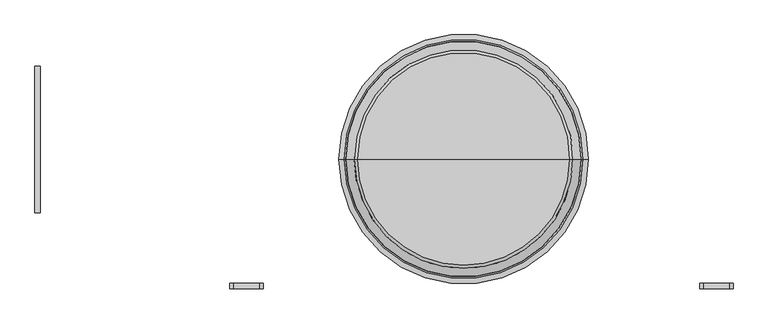
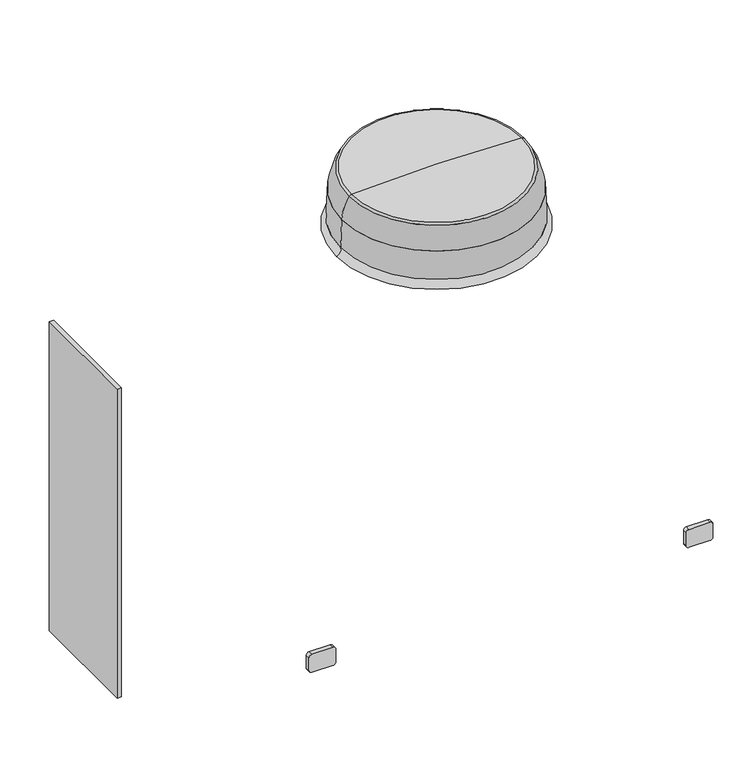
"""IFC4 building model written with IfcOpenShell, lengths in millimetres: proxy geometry, PURY-P168-288_YSJMU_Heat_Recovery_460V : PURY-P192YSJMU-A(-BS)_460V."""

import ifcopenshell
import ifcopenshell.guid

model = None  # the IFC model being written
_history = None  # IfcOwnerHistory: only IFC2X3 demands one
_inside = {}  # id of a spatial element -> (the spatial element, [elements in it])
_under = {}  # id of a project, library or spatial element -> (it, [spatial elements below it])
_declared = {}  # id of a project -> (the project, [libraries it declares])
_typed = {}  # id of a type object -> (the type object, [elements of that type])
_made_of = {}  # id of a material, layer set ... -> (it, [elements and type objects made of it])


def new_model(schema):
    """Start an empty IFC model of exactly this schema.

    Asked for "IFC4X3", IfcOpenShell would pick the latest addendum, in which some entities
    have other attributes; the version numbers below select the first issue.
    IFC2X3 requires an IfcOwnerHistory on every rooted entity: one is made here for all.
    """
    global model, _history
    if schema == "IFC4X3":
        model = ifcopenshell.file(schema_version=(4, 3, 0, 0))
    else:
        model = ifcopenshell.file(schema=schema)
    _inside.clear()
    _under.clear()
    _declared.clear()
    _typed.clear()
    _made_of.clear()
    _history = None
    if model.schema == "IFC2X3":
        org = make("IfcOrganization", Name="unknown")
        user = make(
            "IfcPersonAndOrganization",
            ThePerson=make("IfcPerson", FamilyName="unknown"),
            TheOrganization=org,
        )
        app = make(
            "IfcApplication",
            ApplicationDeveloper=org,
            Version="unknown",
            ApplicationFullName="unknown",
            ApplicationIdentifier="unknown",
        )
        _history = make(
            "IfcOwnerHistory",
            OwningUser=user,
            OwningApplication=app,
            ChangeAction="ADDED",
            CreationDate=0,
        )
    return model


def make(cls, **values):
    """One entity of the class cls with the attributes given. An attribute that is None is left unset."""
    return model.create_entity(
        cls, **{name: value for name, value in values.items() if value is not None}
    )


def rooted(cls, **values):
    """An entity with a GlobalId (a new one), such as an element, a storey or a relation."""
    return make(cls, GlobalId=ifcopenshell.guid.new(), OwnerHistory=_history, **values)


def si_unit(unit_type, name, prefix=None):
    """IfcSIUnit, for example si_unit("LENGTHUNIT", "METRE", prefix="MILLI")."""
    return make("IfcSIUnit", UnitType=unit_type, Prefix=prefix, Name=name)


def assignment(units):
    """IfcUnitAssignment: the units of a project."""
    return None if units is None else make("IfcUnitAssignment", Units=units)


def point(xyz):
    """IfcCartesianPoint."""
    return None if xyz is None else make("IfcCartesianPoint", Coordinates=xyz)


def direction(xyz):
    """IfcDirection."""
    return None if xyz is None else make("IfcDirection", DirectionRatios=xyz)


def frame(location, z_axis=None, x_axis=None):
    """IfcAxis2Placement3D, a coordinate frame: its origin and axes. An axis left out is left unset."""
    return make(
        "IfcAxis2Placement3D",
        Location=point(location),
        Axis=direction(z_axis),
        RefDirection=direction(x_axis),
    )


def frame_2d(location, x_axis=None):
    """IfcAxis2Placement2D, a coordinate frame in the plane: its origin and x axis."""
    return make(
        "IfcAxis2Placement2D", Location=point(location), RefDirection=direction(x_axis)
    )


def origin():
    """The frame at (0, 0, 0) with its axes left unset."""
    return frame((0.0, 0.0, 0.0))


def place(relative_to, where):
    """IfcLocalPlacement: puts the frame where relative to a parent placement (None: the world)."""
    return make(
        "IfcLocalPlacement", PlacementRelTo=relative_to, RelativePlacement=where
    )


def context(
    kind, dimensions, precision=None, world=None, true_north=None, identifier=None
):
    """IfcGeometricRepresentationContext, for example the 3D "Model" context."""
    return make(
        "IfcGeometricRepresentationContext",
        ContextIdentifier=identifier,
        ContextType=kind,
        CoordinateSpaceDimension=dimensions,
        Precision=precision,
        WorldCoordinateSystem=world,
        TrueNorth=true_north,
    )


def project(units=None, contexts=None):
    """IfcProject with its units and contexts."""
    return rooted(
        "IfcProject",
        Name="project",
        RepresentationContexts=contexts,
        UnitsInContext=assignment(units),
    )


def spatial(cls, under=None, at=None, **own):
    """A site, building, storey or space (cls), placed at a placement, below another one or the project."""
    s = rooted(cls, ObjectPlacement=at, **own)
    if under is not None:
        _under.setdefault(under.id(), (under, []))[1].append(s)
    return s


def polyline(points):
    """IfcPolyline through the points."""
    return make("IfcPolyline", Points=[point(p) for p in points])


def circle_curve(where, radius):
    """IfcCircle in the frame where."""
    return make("IfcCircle", Position=where, Radius=radius)


def ellipse_curve(where, semi_axis1, semi_axis2):
    """IfcEllipse in the frame where."""
    return make(
        "IfcEllipse", Position=where, SemiAxis1=semi_axis1, SemiAxis2=semi_axis2
    )


def trimmed(basis, trim1, trim2, sense, master):
    """IfcTrimmedCurve: the piece of a basis curve between two trims."""
    return make(
        "IfcTrimmedCurve",
        BasisCurve=basis,
        Trim1=trim1,
        Trim2=trim2,
        SenseAgreement=sense,
        MasterRepresentation=master,
    )


def segment(curve, same_sense, transition):
    """IfcCompositeCurveSegment."""
    return make(
        "IfcCompositeCurveSegment",
        Transition=transition,
        SameSense=same_sense,
        ParentCurve=curve,
    )


def composite_curve(segments, self_intersect=None):
    """IfcCompositeCurve: segments joined end to end."""
    return make("IfcCompositeCurve", Segments=segments, SelfIntersect=self_intersect)


def outline(outer, holes=None, kind="AREA"):
    """IfcArbitraryClosedProfileDef: a profile drawn as a closed curve; with holes, ...WithVoids."""
    if holes is None:
        return make("IfcArbitraryClosedProfileDef", ProfileType=kind, OuterCurve=outer)
    return make(
        "IfcArbitraryProfileDefWithVoids",
        ProfileType=kind,
        OuterCurve=outer,
        InnerCurves=holes,
    )


def extrude(swept, where, along, depth):
    """IfcExtrudedAreaSolid: the profile swept, set in the frame where, extruded along a direction by depth."""
    return make(
        "IfcExtrudedAreaSolid",
        SweptArea=swept,
        Position=where,
        ExtrudedDirection=direction(along),
        Depth=depth,
    )


def shape(context_of_items, identifier, shape_type, items):
    """IfcShapeRepresentation: the items that make up one representation, for example the "Body"."""
    return make(
        "IfcShapeRepresentation",
        ContextOfItems=context_of_items,
        RepresentationIdentifier=identifier,
        RepresentationType=shape_type,
        Items=items,
    )


def source(mapping_origin, context_of_items, identifier, shape_type, items):
    """IfcRepresentationMap: a shape defined once, which mapped items show again and again."""
    return make(
        "IfcRepresentationMap",
        MappingOrigin=mapping_origin,
        MappedRepresentation=shape(context_of_items, identifier, shape_type, items),
    )


def transform(
    local_origin,
    x_axis=None,
    y_axis=None,
    z_axis=None,
    scale=None,
    scale2=None,
    scale3=None,
    uniform=True,
):
    """IfcCartesianTransformationOperator3D, or its non-uniform kind. x_axis, y_axis, z_axis: its Axis1, 2, 3."""
    if uniform:
        return make(
            "IfcCartesianTransformationOperator3D",
            Axis1=direction(x_axis),
            Axis2=direction(y_axis),
            LocalOrigin=point(local_origin),
            Scale=scale,
            Axis3=direction(z_axis),
        )
    return make(
        "IfcCartesianTransformationOperator3DnonUniform",
        Axis1=direction(x_axis),
        Axis2=direction(y_axis),
        LocalOrigin=point(local_origin),
        Scale=scale,
        Axis3=direction(z_axis),
        Scale2=scale2,
        Scale3=scale3,
    )


def mapped(mapping_source, mapping_target):
    """IfcMappedItem: shows the shape of a source again, moved by a transform."""
    return make(
        "IfcMappedItem", MappingSource=mapping_source, MappingTarget=mapping_target
    )


def made_of(thing, what):
    """Note that an element or type object is made of a material, layer set ...; save() writes the relation."""
    if what is not None:
        _made_of.setdefault(what.id(), (what, []))[1].append(thing)
    return thing


def element(
    cls,
    number,
    at=None,
    inside=None,
    cuts=None,
    type_object=None,
    material=None,
    context=None,
    identifier="Body",
    shape_type=None,
    held_by="IfcProductDefinitionShape",
    body=None,
    shapes=None,
    **own,
):
    """One element of the class cls, such as IfcWall. Its Tag is "e" and its number.

    at: its placement. inside: the storey or other place that contains it. cuts: it is an
    opening in that element (IfcRelVoidsElement). A single representation is given by context,
    identifier, shape_type and body (its items); several are given by shapes. held_by: the class
    of the entity that holds the representations. save() writes the other relations.
    """
    e = rooted(cls, Tag="e%d" % number, ObjectPlacement=at, **own)
    if body is not None:
        shapes = [shape(context, identifier, shape_type, body)]
    if shapes is not None:
        e.Representation = make(held_by, Representations=shapes)
    if inside is not None:
        _inside.setdefault(inside.id(), (inside, []))[1].append(e)
    if cuts is not None:
        rooted(
            "IfcRelVoidsElement", RelatingBuildingElement=cuts, RelatedOpeningElement=e
        )
    if type_object is not None:
        _typed.setdefault(type_object.id(), (type_object, []))[1].append(e)
    return made_of(e, material)


def aggregate(whole, parts):
    """IfcRelAggregates: a whole, such as a stair, and the parts it consists of."""
    return rooted("IfcRelAggregates", RelatingObject=whole, RelatedObjects=parts)


def save(model, path):
    """Write the relations noted so far, then the file.

    IfcRelAggregates (storeys below a building ...), IfcRelContainedInSpatialStructure (elements
    in a storey), IfcRelDefinesByType, IfcRelAssociatesMaterial and IfcRelDeclares: one each for
    every whole, place, type object, material and project.
    """
    for whole, parts in _under.values():
        aggregate(whole, parts)
    for where, things in _inside.values():
        rooted(
            "IfcRelContainedInSpatialStructure",
            RelatedElements=things,
            RelatingStructure=where,
        )
    for kind, things in _typed.values():
        rooted("IfcRelDefinesByType", RelatedObjects=things, RelatingType=kind)
    for what, things in _made_of.values():
        rooted("IfcRelAssociatesMaterial", RelatedObjects=things, RelatingMaterial=what)
    for by, libraries in _declared.values():
        rooted("IfcRelDeclares", RelatingContext=by, RelatedDefinitions=libraries)
    model.write(path)


def plane_surface(at):
    """IfcPlane: the flat surface through the origin of the frame at, square to its z axis."""
    return make("IfcPlane", Position=at)


def revolved_surface(curve, axis_point, axis_direction):
    """IfcSurfaceOfRevolution: the curve turned about the line through axis_point along axis_direction."""
    return make(
        "IfcSurfaceOfRevolution",
        SweptCurve=make("IfcArbitraryOpenProfileDef", ProfileType="CURVE", Curve=curve),
        AxisPosition=make("IfcAxis1Placement", Location=point(axis_point), Axis=direction(axis_direction)),
    )


def advanced_brep(points, edges, surfaces, faces):
    """IfcAdvancedBrep: a solid bounded by faces that lie on surfaces and meet in shared edges.

    An edge is (start, end): straight between two places in points (the first is 0);
    or (start, end, curve); or (start, end, curve, False) where it runs against its curve.
    A face is (place in surfaces, loops), or (place, loops, False) where it looks against
    its surface's normal. A loop lists edges by number (the first is 1), with a minus sign
    where the edge is run from its end to its start. The first loop is the outer one.
    """
    corners = [point(p) for p in points]
    vertices = [make("IfcVertexPoint", VertexGeometry=c) for c in corners]
    made = []
    for start, end, *more in edges:
        made.append(
            make(
                "IfcEdgeCurve",
                EdgeStart=vertices[start],
                EdgeEnd=vertices[end],
                EdgeGeometry=more[0] if more else make("IfcPolyline", Points=[corners[start], corners[end]]),
                SameSense=more[1] if len(more) > 1 else True,
            )
        )
    hull = []
    for where, loops, *sense in faces:
        bounds = []
        for j, loop in enumerate(loops):
            ring = [make("IfcOrientedEdge", EdgeElement=made[abs(k) - 1], Orientation=k > 0) for k in loop]
            bounds.append(
                make(
                    "IfcFaceOuterBound" if j == 0 else "IfcFaceBound",
                    Bound=make("IfcEdgeLoop", EdgeList=ring),
                    Orientation=True,
                )
            )
        hull.append(make("IfcAdvancedFace", Bounds=bounds, FaceSurface=surfaces[where], SameSense=sense[0] if sense else True))
    return make("IfcAdvancedBrep", Outer=make("IfcClosedShell", CfsFaces=hull))


def mechanical_equipment_79fc2163(model_context):
    return source(origin(), model_context, "Body", "SolidModel", [
        extrude(outline(polyline([(-748.962, -164.0), (-748.962, 284.0), (-732.962, 284.0), (-732.962, -164.0), (-748.962, -164.0)])), frame((0.0, 0.0, 54.0), z_axis=(0.0, 0.0, 1.0), x_axis=(1.0, 0.0, 0.0)), (0.0, 0.0, 1.0), 1245.8),
        advanced_brep(
        [(202.9156536, 0.0, 1550.0000157), (924.1603464, 0.0, 1550.0000157), (563.538, 0.0, 1550.0000157), (228.7569245, 0.0, 1635.7196156), (898.3190755, 0.0, 1635.7196156), (237.9260831, 0.0, 1640.2981249), (889.1499169, 0.0, 1640.2981249), (563.538, 0.0, 1649.7941679)],
        [
            (0, 1, circle_curve(frame((563.538, 0.0, 1550.0000157), z_axis=(0.0, 0.0, -1.0), x_axis=(1.0, 0.0, 0.0)), 360.6223464)),
            (1, 2),
            (2, 0),
            (1, 0, circle_curve(frame((563.538, 0.0, 1550.0000157), z_axis=(0.0, 0.0, -1.0), x_axis=(1.0, 0.0, 0.0)), 360.6223464)),
            (3, 4, circle_curve(frame((563.538, 0.0, 1635.7196156), z_axis=(0.0, 0.0, -1.0), x_axis=(1.0, 0.0, 0.0)), 334.7810755)),
            (4, 1, circle_curve(frame((740.2568175, 0.0, 1541.3148332), z_axis=(0.0, 1.0, 0.0), x_axis=(1.0, 0.0, 0.0)), 184.1085015)),
            (0, 3, circle_curve(frame((386.8191825, 0.0, 1541.3148332), z_axis=(0.0, 1.0, 0.0), x_axis=(-1.0, 0.0, 0.0)), 184.1085015)),
            (4, 3, circle_curve(frame((563.538, 0.0, 1635.7196156), z_axis=(0.0, 0.0, -1.0), x_axis=(1.0, 0.0, 0.0)), 334.7810755)),
            (5, 6, circle_curve(frame((563.538, 0.0, 1640.2981249), z_axis=(0.0, 0.0, -1.0), x_axis=(1.0, 0.0, 0.0)), 325.6119169)),
            (6, 4, circle_curve(frame((889.1499169, 0.0, 1628.8275558), z_axis=(0.0, 1.0, 0.0), x_axis=(1.0, 0.0, 0.0)), 11.4705691)),
            (3, 5, circle_curve(frame((237.9260831, 0.0, 1628.8275558), z_axis=(0.0, 1.0, 0.0), x_axis=(-1.0, 0.0, 0.0)), 11.4705691)),
            (6, 5, circle_curve(frame((563.538, 0.0, 1640.2981249), z_axis=(0.0, 0.0, -1.0), x_axis=(1.0, 0.0, 0.0)), 325.6119169)),
            (7, 6, circle_curve(frame((563.538, 0.0, -3937.4433334), z_axis=(0.0, 1.0, 0.0), x_axis=(1.0, 0.0, 0.0)), 5587.2375013)),
            (5, 7, circle_curve(frame((563.538, 0.0, -3937.4433334), z_axis=(0.0, 1.0, 0.0), x_axis=(-1.0, 0.0, 0.0)), 5587.2375013)),
        ],
        [
            plane_surface(frame((563.538, 0.0, 1550.0000157), z_axis=(0.0, 0.0, -1.0), x_axis=(1.0, 0.0, 0.0))),
            revolved_surface(trimmed(ellipse_curve(frame((740.2568175, 0.0, 1541.3148332), z_axis=(0.0, -1.0, 0.0), x_axis=(1.0, 0.0, 0.0)), 184.1085015, 184.1085015), [point((924.1603464, 0.0, 1550.0000157))], [point((898.3190755, 0.0, 1635.7196156))], True, "CARTESIAN"), (563.538, 0.0, 1605.0), (0.0, 0.0, 1.0)),
            revolved_surface(trimmed(ellipse_curve(frame((889.1499169, 0.0, 1628.8275558), z_axis=(0.0, -1.0, 0.0), x_axis=(1.0, 0.0, 0.0)), 11.4705691, 11.4705691), [point((898.3190755, 0.0, 1635.7196156))], [point((889.1499169, 0.0, 1640.2981249))], True, "CARTESIAN"), (563.538, 0.0, 1605.0), (0.0, 0.0, 1.0)),
            revolved_surface(trimmed(ellipse_curve(frame((563.538, 0.0, -3937.4433334), z_axis=(0.0, -1.0, 0.0), x_axis=(1.0, 0.0, 0.0)), 5587.2375013, 5587.2375013), [point((889.1499169, 0.0, 1640.2981249))], [point((563.538, 0.0, 1649.7941679))], True, "CARTESIAN"), (563.538, 0.0, 1605.0), (0.0, 0.0, 1.0)),
        ],
        [
            (0, [[1, 2, 3]]),
            (0, [[4, -3, -2]]),
            (1, [[5, 6, -1, 7]]),
            (1, [[8, -7, -4, -6]]),
            (2, [[9, 10, -5, 11]]),
            (2, [[12, -11, -8, -10]]),
            (3, [[13, -9, 14]]),
            (3, [[-14, -12, -13]]),
        ],
    ),
        advanced_brep(
        [(181.4881528, 0.0, 1410.0), (945.5878472, 0.0, 1410.0), (563.538, 0.0, 1410.0), (198.0531583, 0.0, 1438.6914312), (929.0228417, 0.0, 1438.6914312), (202.9129453, 0.0, 1550.0000157), (924.1630547, 0.0, 1550.0000157), (563.538, 0.0, 1550.0000157)],
        [
            (0, 1, circle_curve(frame((563.538, 0.0, 1410.0), z_axis=(0.0, 0.0, -1.0), x_axis=(1.0, 0.0, 0.0)), 382.0498472)),
            (1, 2),
            (2, 0),
            (1, 0, circle_curve(frame((563.538, 0.0, 1410.0), z_axis=(0.0, 0.0, -1.0), x_axis=(1.0, 0.0, 0.0)), 382.0498472)),
            (3, 4, circle_curve(frame((563.538, 0.0, 1438.6914312), z_axis=(0.0, 0.0, -1.0), x_axis=(1.0, 0.0, 0.0)), 365.4848417)),
            (4, 1, circle_curve(frame((949.7748091, 0.0, 1431.5449644), z_axis=(0.0, -1.0, 0.0), x_axis=(1.0, 0.0, 0.0)), 21.9480327)),
            (0, 3, circle_curve(frame((177.3011909, 0.0, 1431.5449644), z_axis=(0.0, -1.0, 0.0), x_axis=(-1.0, 0.0, 0.0)), 21.9480327)),
            (4, 3, circle_curve(frame((563.538, 0.0, 1438.6914312), z_axis=(0.0, 0.0, -1.0), x_axis=(1.0, 0.0, 0.0)), 365.4848417)),
            (5, 6, circle_curve(frame((563.538, 0.0, 1550.0000157), z_axis=(0.0, 0.0, -1.0), x_axis=(1.0, 0.0, 0.0)), 360.6250547)),
            (6, 4),
            (3, 5),
            (6, 5, circle_curve(frame((563.538, 0.0, 1550.0000157), z_axis=(0.0, 0.0, -1.0), x_axis=(1.0, 0.0, 0.0)), 360.6250547)),
            (7, 6),
            (5, 7),
        ],
        [
            plane_surface(frame((563.538, 0.0, 1410.0), z_axis=(0.0, 0.0, -1.0), x_axis=(1.0, 0.0, 0.0))),
            revolved_surface(trimmed(ellipse_curve(frame((949.7748091, 0.0, 1431.5449644), z_axis=(0.0, 1.0, 0.0), x_axis=(1.0, 0.0, 0.0)), 21.9480327, 21.9480327), [point((945.5878472, 0.0, 1410.0))], [point((929.0228417, 0.0, 1438.6914312))], True, "CARTESIAN"), (563.538, 0.0, 1470.0), (0.0, 0.0, 1.0)),
            revolved_surface(polyline([(929.0228417, 0.0, 1438.6914312), (924.1630547, 0.0, 1550.0000157)]), (563.538, 0.0, 1470.0), (0.0, 0.0, 1.0)),
            plane_surface(frame((563.538, 0.0, 1550.0000157), z_axis=(0.0, 0.0, 1.0), x_axis=(1.0, 0.0, 0.0))),
        ],
        [
            (0, [[1, 2, 3]]),
            (0, [[4, -3, -2]]),
            (1, [[5, 6, -1, 7]]),
            (1, [[8, -7, -4, -6]]),
            (2, [[9, 10, -5, 11]]),
            (2, [[12, -11, -8, -10]]),
            (3, [[13, -9, 14]]),
            (3, [[-14, -12, -13]]),
        ],
    ),
        extrude(outline(composite_curve([segment(trimmed(circle_curve(frame_2d((148.5853631, 1296.6117511)), 9.9920268), [point((158.5773899, 1296.6117511))], [point((148.5853631, 1286.6197243))], False, "CARTESIAN"), True, "CONTINUOUS"), segment(polyline([(148.5853631, 1286.6197243), (96.5694168, 1286.6197243)]), True, "CONTINUOUS"), segment(trimmed(circle_curve(frame_2d((96.5694168, 1296.6117511)), 9.9920268), [point((96.5694168, 1286.6197243))], [point((86.5773899, 1296.6117511))], False, "CARTESIAN"), True, "CONTINUOUS"), segment(polyline([(86.5773899, 1296.6117511), (86.5773899, 1378.6276974)]), True, "CONTINUOUS"), segment(trimmed(circle_curve(frame_2d((96.5694168, 1378.6276974)), 9.9920268), [point((86.5773899, 1378.6276974))], [point((96.5694168, 1388.6197243))], False, "CARTESIAN"), True, "CONTINUOUS"), segment(polyline([(96.5694168, 1388.6197243), (148.5853631, 1388.6197243)]), True, "CONTINUOUS"), segment(trimmed(circle_curve(frame_2d((148.5853631, 1378.6276974)), 9.9920268), [point((148.5853631, 1388.6197243))], [point((158.5773899, 1378.6276974))], False, "CARTESIAN"), True, "CONTINUOUS"), segment(polyline([(158.5773899, 1378.6276974), (158.5773899, 1296.6117511)]), True, "CONTINUOUS")], self_intersect=False)), frame((0.0, -397.2710787, 0.0), z_axis=(0.0, 1.0, 0.0), x_axis=(0.0, 0.0, 1.0)), (0.0, 0.0, 1.0), 17.2710787),
        extrude(outline(composite_curve([segment(trimmed(circle_curve(frame_2d((148.5853631, -142.3882489)), 9.9920268), [point((158.5773899, -142.3882489))], [point((148.5853631, -152.3802757))], False, "CARTESIAN"), True, "CONTINUOUS"), segment(polyline([(148.5853631, -152.3802757), (96.5694168, -152.3802757)]), True, "CONTINUOUS"), segment(trimmed(circle_curve(frame_2d((96.5694168, -142.3882489)), 9.9920268), [point((96.5694168, -152.3802757))], [point((86.5773899, -142.3882489))], False, "CARTESIAN"), True, "CONTINUOUS"), segment(polyline([(86.5773899, -142.3882489), (86.5773899, -60.3723026)]), True, "CONTINUOUS"), segment(trimmed(circle_curve(frame_2d((96.5694168, -60.3723026)), 9.9920268), [point((86.5773899, -60.3723026))], [point((96.5694168, -50.3802757))], False, "CARTESIAN"), True, "CONTINUOUS"), segment(polyline([(96.5694168, -50.3802757), (148.5853631, -50.3802757)]), True, "CONTINUOUS"), segment(trimmed(circle_curve(frame_2d((148.5853631, -60.3723026)), 9.9920268), [point((148.5853631, -50.3802757))], [point((158.5773899, -60.3723026))], False, "CARTESIAN"), True, "CONTINUOUS"), segment(polyline([(158.5773899, -60.3723026), (158.5773899, -142.3882489)]), True, "CONTINUOUS")], self_intersect=False)), frame((0.0, -397.2710787, 0.0), z_axis=(0.0, 1.0, 0.0), x_axis=(0.0, 0.0, 1.0)), (0.0, 0.0, 1.0), 17.2710787),
    ])


if __name__ == "__main__":
    model = new_model("IFC4")
    model_context = context("Model", 3, world=origin())
    ifc_project = project(units=[si_unit("LENGTHUNIT", "METRE", prefix="MILLI")], contexts=[model_context])
    site = spatial("IfcSite", under=ifc_project)
    building = spatial("IfcBuilding", under=site)
    placement = place(None, origin())
    mechanical_equipment_shape = mechanical_equipment_79fc2163(model_context)
    element("IfcBuildingElementProxy", 1, Name="PURY-P168-288_YSJMU_Heat_Recovery_460V : PURY-P192YSJMU-A(-BS)_460V", ObjectType="PURY-P168-288_YSJMU_Heat_Recovery_460V : PURY-P192YSJMU-A(-BS)_460V", at=placement, inside=building, context=model_context, shape_type="MappedRepresentation", body=[
        mapped(mechanical_equipment_shape, transform((0.0, 0.0, 0.0), x_axis=(1.0, 0.0, 0.0), y_axis=(0.0, 1.0, 0.0), z_axis=(0.0, 0.0, 1.0))),
    ])
    save(model, "model.ifc")

# Revit data of these elements
# Type "PURY-P168-288_YSJMU_Heat_Recovery_460V : PURY-P192YSJMU-A(-BS)_460V"
#   Unit Weight (LBS) = "618 x 2"
#   Technical and Installation = "http://www.mrslim.com/customerCare/resources.asp"
#   Specification URL = "http://www.mrslim.com/customerCare/resources.asp"
#   Sound Pressure Levels (dB(A)) = "61"
#   SmartBIM Object Created By = "Reed Construction Data"
#   Refrigerant Type = "R410A"
#   Refrigerant Charge = ""
#   Recommended Breaker Size = "25 A x 1 + 15 A x 1"
#   Protection Devices Inverter = "Overheat / Overcurrent Protection"
#   Protection Devices High Pressure = "601 psi / 4.15 MPa"
#   Protection Devices Fan = "Overheat Protection / Thermal Switch"
#   Protection Devices Compressor = "Overheat Protection / Thermal Switch"
#   Product URL = "http://www.mrslim.com/customerCare/resources.asp"
#   Power Source = "208 / 230V, 3-phase, 60Hz"
#   Power Input Heating = "16.07 kW"
#   Power Input Cooling = "17.84 kW"
#   URL = "http://www.mehvac.com"
#   OmniClass Code = "22-23 81 26"
#   MOCP = "30 A x 1 + 15 A x 1"
#   MCA = "23 A x 1 + 13 A x 1"
#   Lubricant = "MEL32"
#   Installation URL = "http://www.mrslim.com/customerCare/resources.asp"
#   Heating Outdoor = "-4° ~ +60°F (-20° ~ +16°C) WB"
#   Heating Indoor = "59° ~ 81°F (15° ~ 27°C) DB"
#   Heating Capacity(BTU) = "215,000"
#   Fan Type x Quantity = "Propeller Fan x 3"
#   Fan Motor Output = "0.92 kW x 3"
#   Fan Air Flow Rate = "10,600 CFM x 1 / 6,180 CFM x 1"
#   Model = "PURY-P192YSJMU-A(-BS)_460V"
#   Manufacturer = "Mitsubishi Electric"
#   Current Heating = "28.2 A"
#   Current Cooling = "25.5 A"
#   Cooling Outdoor = "23° ~ 115°F (-5° ~ +46°C) DB"
#   Cooling Indoor = "59° ~ 75°F (15° ~ +24°C) WB"
#   Cooling Capacity (BTU) = "192,000"
#   Compressor Type x Quantity = "Inverter-driven Scroll Hermetic x 1 for Each Module"
#   Compressor Operating Range = "8% to 100%"
#   Case Heater = "0.045 kW"
#   Assembly Code = "D3090100"
#   95 CSI = "15740"
#   04 CSI = "23 81 26"
#   Voltage = 208 V
#   SmartBIM Object Version = 3
#   Refrigerant Pipe diameter (low pressure) = 0' - 1 1/8"
#   Refrigerant Pipe diameter (high pressure) = 0' - 0 7/8"
#   Phase = 3
#   Outdoor Unit2-Width = 3' - 0.22047"
#   Outdoor Unit1-Width = 5' - 8.89764"
#   Offset = 0' - 1.1811"
#   Hertz = 60
#   Height = 5' - 4.96063"
#   Depth = 2' - 5.92126"
#   Apparent Load = 19871 VA
#   Number of Poles = 2
#   Load Classification = HVAC
#   External Material = Pre-coated Galvanized-steel Sheets
#   External Finish = Pre-coated Galvanized-steel Sheets
#   Air Outlet Unit Material = Metal Grille
#   Air Inlet Unit Material = Grille
#   Type Comments = ""
#   Description = (empty or 0)
#   Default Elevation = 0
# Element 1 (IfcBuildingElementProxy, "PURY-P168-288_YSJMU_Heat_Recovery_460V : PURY-P192YSJMU-A(-BS)_460V")
#   Materials on its faces: "Pre-coated Galvanized-steel Sheets", "Grille", "Metal Grille"
# Materials
#   "Pre-coated Galvanized-steel Sheets": class "Metal", colour RGB 189 187 185, transparency 0
#   "Metal Grille": class "Metal", colour RGB 10 10 10, transparency 0
#   "Grille": class "Miscellaneous", colour RGB 0 0 0, transparency 0
